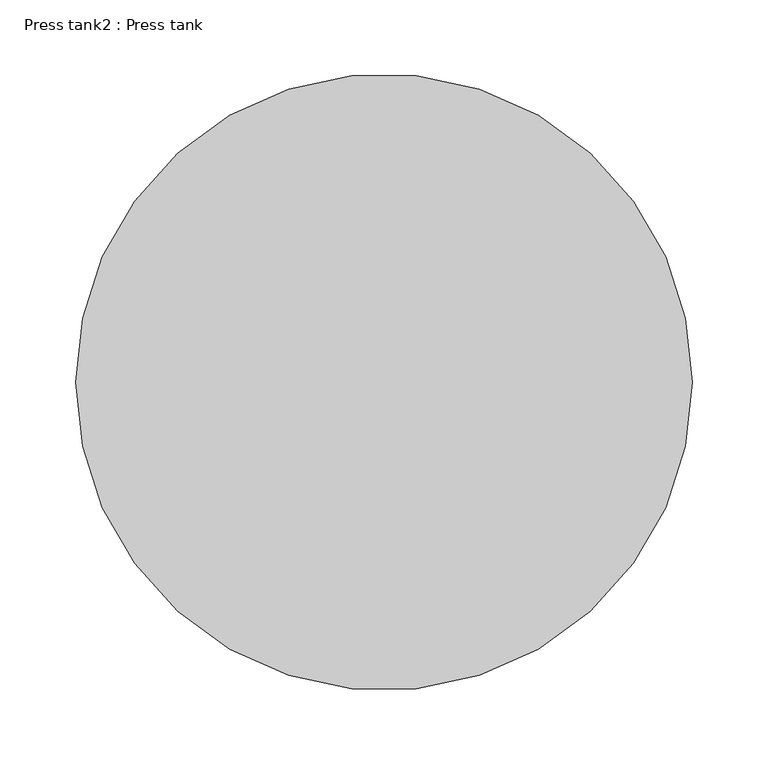
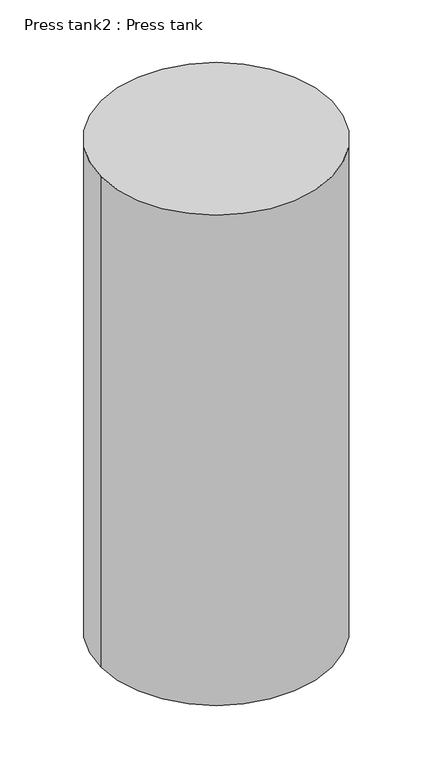
"""IFC4 building model written with IfcOpenShell, lengths in millimetres: proxy geometry, Press tank2 : Press tank."""

from ifc_helpers import new_model, si_unit, point, frame, frame_2d, origin, place, context, project, spatial, circle_curve, trimmed, segment, composite_curve, outline, extrude, source, transform, mapped, element, save


def press_tank2_press_tank_b5f43448(model_context):
    return source(origin(), model_context, "Body", "SweptSolid", [
        extrude(outline(composite_curve([segment(trimmed(circle_curve(frame_2d((23819.6370052, 10524.1286841)), 203.2), [point((23616.4370052, 10524.1286841))], [point((24022.8370052, 10524.1286841))], False, "CARTESIAN"), True, "CONTINUOUS"), segment(trimmed(circle_curve(frame_2d((23819.6370052, 10524.1286841)), 203.2), [point((24022.8370052, 10524.1286841))], [point((23616.4370052, 10524.1286841))], False, "CARTESIAN"), True, "CONTINUOUS")], self_intersect=False)), frame((0.0, 0.0, 2832.1), z_axis=(0.0, 0.0, 1.0), x_axis=(1.0, 0.0, 0.0)), (0.0, 0.0, 1.0), 914.4),
    ])


if __name__ == "__main__":
    model = new_model("IFC4")
    model_context = context("Model", 3, world=origin())
    ifc_project = project(units=[si_unit("LENGTHUNIT", "METRE", prefix="MILLI")], contexts=[model_context])
    site = spatial("IfcSite", under=ifc_project)
    building = spatial("IfcBuilding", under=site)
    placement = place(None, origin())
    press_tank2_press_tank_shape = press_tank2_press_tank_b5f43448(model_context)
    element("IfcBuildingElementProxy", 1, Name="Press tank2 : Press tank", ObjectType="Press tank2 : Press tank", at=placement, inside=building, context=model_context, shape_type="MappedRepresentation", body=[
        mapped(press_tank2_press_tank_shape, transform((0.0, 0.0, 0.0), x_axis=(1.0, 0.0, 0.0), y_axis=(0.0, 1.0, 0.0), z_axis=(0.0, 0.0, 1.0))),
    ])
    save(model, "model.ifc")
